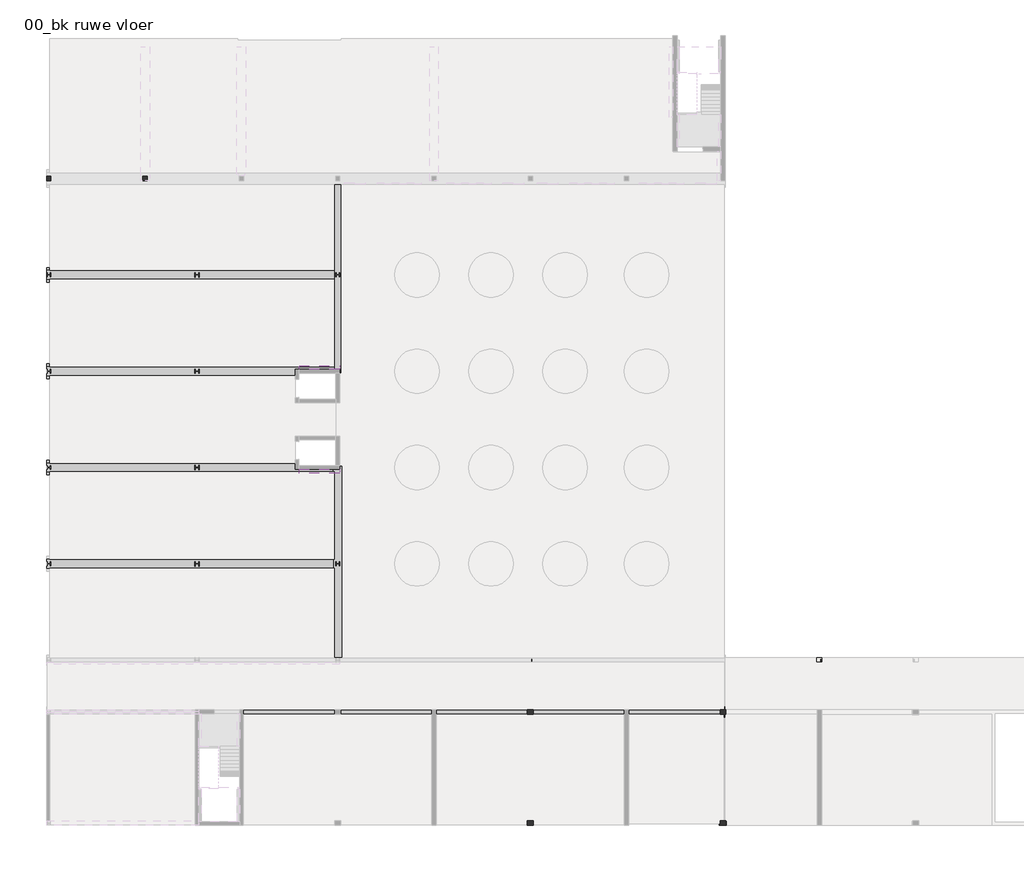
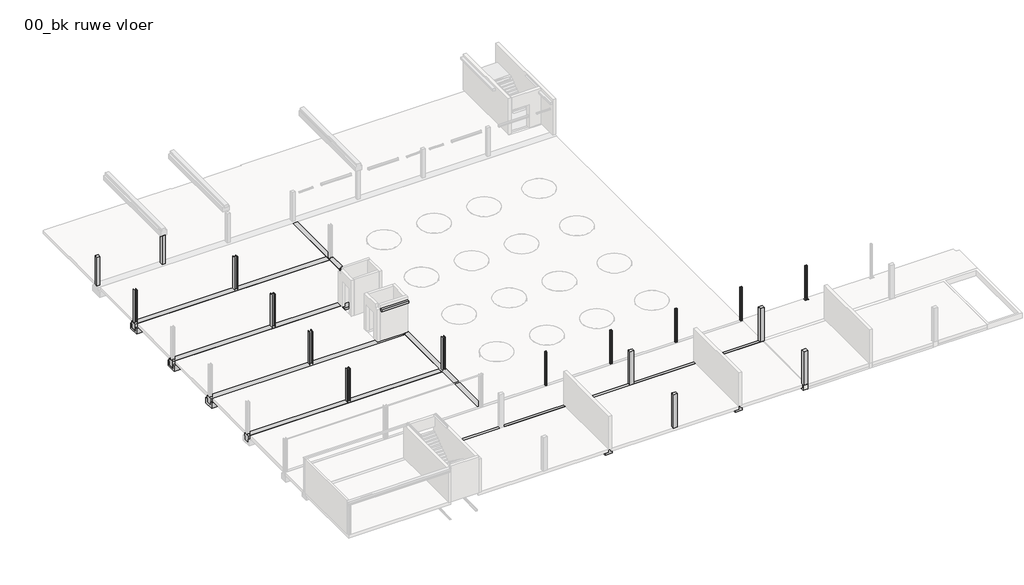
# One storey, part 5 of 6: 17 columns, 14 beams, 2 slabs.
"""IFC4 building model written with IfcOpenShell, lengths in millimetres."""

import ifcopenshell
import ifcopenshell.guid

model = None  # the IFC model being written
_history = None  # IfcOwnerHistory: only IFC2X3 demands one
_inside = {}  # id of a spatial element -> (the spatial element, [elements in it])
_under = {}  # id of a project, library or spatial element -> (it, [spatial elements below it])
_declared = {}  # id of a project -> (the project, [libraries it declares])
_typed = {}  # id of a type object -> (the type object, [elements of that type])
_made_of = {}  # id of a material, layer set ... -> (it, [elements and type objects made of it])


def new_model(schema):
    """Start an empty IFC model of exactly this schema.

    Asked for "IFC4X3", IfcOpenShell would pick the latest addendum, in which some entities
    have other attributes; the version numbers below select the first issue.
    IFC2X3 requires an IfcOwnerHistory on every rooted entity: one is made here for all.
    """
    global model, _history
    if schema == "IFC4X3":
        model = ifcopenshell.file(schema_version=(4, 3, 0, 0))
    else:
        model = ifcopenshell.file(schema=schema)
    _inside.clear()
    _under.clear()
    _declared.clear()
    _typed.clear()
    _made_of.clear()
    _history = None
    if model.schema == "IFC2X3":
        org = make("IfcOrganization", Name="unknown")
        user = make(
            "IfcPersonAndOrganization",
            ThePerson=make("IfcPerson", FamilyName="unknown"),
            TheOrganization=org,
        )
        app = make(
            "IfcApplication",
            ApplicationDeveloper=org,
            Version="unknown",
            ApplicationFullName="unknown",
            ApplicationIdentifier="unknown",
        )
        _history = make(
            "IfcOwnerHistory",
            OwningUser=user,
            OwningApplication=app,
            ChangeAction="ADDED",
            CreationDate=0,
        )
    return model


def make(cls, **values):
    """One entity of the class cls with the attributes given. An attribute that is None is left unset."""
    return model.create_entity(
        cls, **{name: value for name, value in values.items() if value is not None}
    )


def rooted(cls, **values):
    """An entity with a GlobalId (a new one), such as an element, a storey or a relation."""
    return make(cls, GlobalId=ifcopenshell.guid.new(), OwnerHistory=_history, **values)


def si_unit(unit_type, name, prefix=None):
    """IfcSIUnit, for example si_unit("LENGTHUNIT", "METRE", prefix="MILLI")."""
    return make("IfcSIUnit", UnitType=unit_type, Prefix=prefix, Name=name)


def assignment(units):
    """IfcUnitAssignment: the units of a project."""
    return None if units is None else make("IfcUnitAssignment", Units=units)


def point(xyz):
    """IfcCartesianPoint."""
    return None if xyz is None else make("IfcCartesianPoint", Coordinates=xyz)


def direction(xyz):
    """IfcDirection."""
    return None if xyz is None else make("IfcDirection", DirectionRatios=xyz)


def frame(location, z_axis=None, x_axis=None):
    """IfcAxis2Placement3D, a coordinate frame: its origin and axes. An axis left out is left unset."""
    return make(
        "IfcAxis2Placement3D",
        Location=point(location),
        Axis=direction(z_axis),
        RefDirection=direction(x_axis),
    )


def frame_2d(location, x_axis=None):
    """IfcAxis2Placement2D, a coordinate frame in the plane: its origin and x axis."""
    return make(
        "IfcAxis2Placement2D", Location=point(location), RefDirection=direction(x_axis)
    )


def origin():
    """The frame at (0, 0, 0) with its axes left unset."""
    return frame((0.0, 0.0, 0.0))


def place(relative_to, where):
    """IfcLocalPlacement: puts the frame where relative to a parent placement (None: the world)."""
    return make(
        "IfcLocalPlacement", PlacementRelTo=relative_to, RelativePlacement=where
    )


def context(
    kind, dimensions, precision=None, world=None, true_north=None, identifier=None
):
    """IfcGeometricRepresentationContext, for example the 3D "Model" context."""
    return make(
        "IfcGeometricRepresentationContext",
        ContextIdentifier=identifier,
        ContextType=kind,
        CoordinateSpaceDimension=dimensions,
        Precision=precision,
        WorldCoordinateSystem=world,
        TrueNorth=true_north,
    )


def project(units=None, contexts=None):
    """IfcProject with its units and contexts."""
    return rooted(
        "IfcProject",
        Name="project",
        RepresentationContexts=contexts,
        UnitsInContext=assignment(units),
    )


def spatial(cls, under=None, at=None, **own):
    """A site, building, storey or space (cls), placed at a placement, below another one or the project."""
    s = rooted(cls, ObjectPlacement=at, **own)
    if under is not None:
        _under.setdefault(under.id(), (under, []))[1].append(s)
    return s


def polyline(points):
    """IfcPolyline through the points."""
    return make("IfcPolyline", Points=[point(p) for p in points])


def circle_curve(where, radius):
    """IfcCircle in the frame where."""
    return make("IfcCircle", Position=where, Radius=radius)


def trimmed(basis, trim1, trim2, sense, master):
    """IfcTrimmedCurve: the piece of a basis curve between two trims."""
    return make(
        "IfcTrimmedCurve",
        BasisCurve=basis,
        Trim1=trim1,
        Trim2=trim2,
        SenseAgreement=sense,
        MasterRepresentation=master,
    )


def segment(curve, same_sense, transition):
    """IfcCompositeCurveSegment."""
    return make(
        "IfcCompositeCurveSegment",
        Transition=transition,
        SameSense=same_sense,
        ParentCurve=curve,
    )


def composite_curve(segments, self_intersect=None):
    """IfcCompositeCurve: segments joined end to end."""
    return make("IfcCompositeCurve", Segments=segments, SelfIntersect=self_intersect)


def outline(outer, holes=None, kind="AREA"):
    """IfcArbitraryClosedProfileDef: a profile drawn as a closed curve; with holes, ...WithVoids."""
    if holes is None:
        return make("IfcArbitraryClosedProfileDef", ProfileType=kind, OuterCurve=outer)
    return make(
        "IfcArbitraryProfileDefWithVoids",
        ProfileType=kind,
        OuterCurve=outer,
        InnerCurves=holes,
    )


def extrude(swept, where, along, depth):
    """IfcExtrudedAreaSolid: the profile swept, set in the frame where, extruded along a direction by depth."""
    return make(
        "IfcExtrudedAreaSolid",
        SweptArea=swept,
        Position=where,
        ExtrudedDirection=direction(along),
        Depth=depth,
    )


def faces_of(points, faces, orient=None, outer=None):
    """IfcFace entities. A face is a list of loops; a loop is a list of indices into points, from 0.

    orient and outer hold one flag for each loop. By default every Orientation is true, the
    first loop of a face is its IfcFaceOuterBound and the others are IfcFaceBound.
    """
    made = []
    for i, loops in enumerate(faces):
        bounds = []
        for j, loop in enumerate(loops):
            is_outer = j == 0 if outer is None else outer[i][j]
            bounds.append(
                make(
                    "IfcFaceOuterBound" if is_outer else "IfcFaceBound",
                    Bound=make("IfcPolyLoop", Polygon=[points[k] for k in loop]),
                    Orientation=True if orient is None else orient[i][j],
                )
            )
        made.append(make("IfcFace", Bounds=bounds))
    return made


def faceted_brep(points, faces, orient=None, outer=None, voids=None):
    """IfcFacetedBrep: a solid bounded by flat faces; with voids (closed shells), ...WithVoids."""
    shared = [point(p) for p in points]
    hull = make("IfcClosedShell", CfsFaces=faces_of(shared, faces, orient, outer))
    if voids is None:
        return make("IfcFacetedBrep", Outer=hull)
    return make(
        "IfcFacetedBrepWithVoids",
        Outer=hull,
        Voids=[
            make(cls, CfsFaces=faces_of(shared, fs, o, b)) for cls, fs, o, b in voids
        ],
    )


def shape(context_of_items, identifier, shape_type, items):
    """IfcShapeRepresentation: the items that make up one representation, for example the "Body"."""
    return make(
        "IfcShapeRepresentation",
        ContextOfItems=context_of_items,
        RepresentationIdentifier=identifier,
        RepresentationType=shape_type,
        Items=items,
    )


def source(mapping_origin, context_of_items, identifier, shape_type, items):
    """IfcRepresentationMap: a shape defined once, which mapped items show again and again."""
    return make(
        "IfcRepresentationMap",
        MappingOrigin=mapping_origin,
        MappedRepresentation=shape(context_of_items, identifier, shape_type, items),
    )


def transform(
    local_origin,
    x_axis=None,
    y_axis=None,
    z_axis=None,
    scale=None,
    scale2=None,
    scale3=None,
    uniform=True,
):
    """IfcCartesianTransformationOperator3D, or its non-uniform kind. x_axis, y_axis, z_axis: its Axis1, 2, 3."""
    if uniform:
        return make(
            "IfcCartesianTransformationOperator3D",
            Axis1=direction(x_axis),
            Axis2=direction(y_axis),
            LocalOrigin=point(local_origin),
            Scale=scale,
            Axis3=direction(z_axis),
        )
    return make(
        "IfcCartesianTransformationOperator3DnonUniform",
        Axis1=direction(x_axis),
        Axis2=direction(y_axis),
        LocalOrigin=point(local_origin),
        Scale=scale,
        Axis3=direction(z_axis),
        Scale2=scale2,
        Scale3=scale3,
    )


def mapped(mapping_source, mapping_target):
    """IfcMappedItem: shows the shape of a source again, moved by a transform."""
    return make(
        "IfcMappedItem", MappingSource=mapping_source, MappingTarget=mapping_target
    )


def made_of(thing, what):
    """Note that an element or type object is made of a material, layer set ...; save() writes the relation."""
    if what is not None:
        _made_of.setdefault(what.id(), (what, []))[1].append(thing)
    return thing


def element(
    cls,
    number,
    at=None,
    inside=None,
    cuts=None,
    type_object=None,
    material=None,
    context=None,
    identifier="Body",
    shape_type=None,
    held_by="IfcProductDefinitionShape",
    body=None,
    shapes=None,
    **own,
):
    """One element of the class cls, such as IfcWall. Its Tag is "e" and its number.

    at: its placement. inside: the storey or other place that contains it. cuts: it is an
    opening in that element (IfcRelVoidsElement). A single representation is given by context,
    identifier, shape_type and body (its items); several are given by shapes. held_by: the class
    of the entity that holds the representations. save() writes the other relations.
    """
    e = rooted(cls, Tag="e%d" % number, ObjectPlacement=at, **own)
    if body is not None:
        shapes = [shape(context, identifier, shape_type, body)]
    if shapes is not None:
        e.Representation = make(held_by, Representations=shapes)
    if inside is not None:
        _inside.setdefault(inside.id(), (inside, []))[1].append(e)
    if cuts is not None:
        rooted(
            "IfcRelVoidsElement", RelatingBuildingElement=cuts, RelatedOpeningElement=e
        )
    if type_object is not None:
        _typed.setdefault(type_object.id(), (type_object, []))[1].append(e)
    return made_of(e, material)


def aggregate(whole, parts):
    """IfcRelAggregates: a whole, such as a stair, and the parts it consists of."""
    return rooted("IfcRelAggregates", RelatingObject=whole, RelatedObjects=parts)


def save(model, path):
    """Write the relations noted so far, then the file.

    IfcRelAggregates (storeys below a building ...), IfcRelContainedInSpatialStructure (elements
    in a storey), IfcRelDefinesByType, IfcRelAssociatesMaterial and IfcRelDeclares: one each for
    every whole, place, type object, material and project.
    """
    for whole, parts in _under.values():
        aggregate(whole, parts)
    for where, things in _inside.values():
        rooted(
            "IfcRelContainedInSpatialStructure",
            RelatedElements=things,
            RelatingStructure=where,
        )
    for kind, things in _typed.values():
        rooted("IfcRelDefinesByType", RelatedObjects=things, RelatingType=kind)
    for what, things in _made_of.values():
        rooted("IfcRelAssociatesMaterial", RelatedObjects=things, RelatingMaterial=what)
    for by, libraries in _declared.values():
        rooted("IfcRelDeclares", RelatingContext=by, RelatedDefinitions=libraries)
    model.write(path)


def column_d8346d76(model_context):
    return source(origin(), model_context, "Body", "SweptSolid", [
        extrude(outline(composite_curve([segment(trimmed(circle_curve(frame_2d((60.0, 60.0)), 20.0), [point((60.0, 80.0))], [point((80.0, 60.0))], False, "CARTESIAN"), True, "CONTINUOUS"), segment(polyline([(80.0, 60.0), (80.0, -60.0)]), True, "CONTINUOUS"), segment(trimmed(circle_curve(frame_2d((60.0, -60.0)), 20.0), [point((80.0, -60.0))], [point((60.0, -80.0))], False, "CARTESIAN"), True, "CONTINUOUS"), segment(polyline([(60.0, -80.0), (-60.0, -80.0)]), True, "CONTINUOUS"), segment(trimmed(circle_curve(frame_2d((-60.0, -60.0)), 20.0), [point((-60.0, -80.0))], [point((-80.0, -60.0))], False, "CARTESIAN"), True, "CONTINUOUS"), segment(polyline([(-80.0, -60.0), (-80.0, 60.0)]), True, "CONTINUOUS"), segment(trimmed(circle_curve(frame_2d((-60.0, 60.0)), 20.0), [point((-80.0, 60.0))], [point((-60.0, 80.0))], False, "CARTESIAN"), True, "CONTINUOUS"), segment(polyline([(-60.0, 80.0), (60.0, 80.0)]), True, "CONTINUOUS")], self_intersect=False), holes=[composite_curve([segment(polyline([(60.0, 72.0), (-60.0, 72.0)]), True, "CONTINUOUS"), segment(trimmed(circle_curve(frame_2d((-60.0, 60.0)), 12.0), [point((-60.0, 72.0))], [point((-72.0, 60.0))], True, "CARTESIAN"), True, "CONTINUOUS"), segment(polyline([(-72.0, 60.0), (-72.0, -60.0)]), True, "CONTINUOUS"), segment(trimmed(circle_curve(frame_2d((-60.0, -60.0)), 12.0), [point((-72.0, -60.0))], [point((-60.0, -72.0))], True, "CARTESIAN"), True, "CONTINUOUS"), segment(polyline([(-60.0, -72.0), (60.0, -72.0)]), True, "CONTINUOUS"), segment(trimmed(circle_curve(frame_2d((60.0, -60.0)), 12.0), [point((60.0, -72.0))], [point((72.0, -60.0))], True, "CARTESIAN"), True, "CONTINUOUS"), segment(polyline([(72.0, -60.0), (72.0, 60.0)]), True, "CONTINUOUS"), segment(trimmed(circle_curve(frame_2d((60.0, 60.0)), 12.0), [point((72.0, 60.0))], [point((60.0, 72.0))], True, "CARTESIAN"), True, "CONTINUOUS")], self_intersect=False)]), frame((0.0, 0.0, -40.0), z_axis=(0.0, 0.0, 1.0), x_axis=(1.0, 0.0, 0.0)), (0.0, 0.0, 1.0), 3510.0),
    ])


model = new_model("IFC4")

# Units and contexts
model_context = context("Model", 3, world=origin())
ifc_project = project(units=[si_unit("LENGTHUNIT", "METRE", prefix="MILLI")], contexts=[model_context])

# Site, building, storey
site = spatial("IfcSite", under=ifc_project)
building = spatial("IfcBuilding", under=site)
storey = spatial("IfcBuildingStorey", under=building, Name="00_bk ruwe vloer", Elevation=-70.0)

# Beams
placement = place(None, origin())
element("IfcBeam", 1, ObjectType="NLRS_28_SF_LIB_balk dubbele sponning beton prefab-CWV-MMBC-SRP_gen_rsf : balk beton prefab_gen__bxh 700x700 met inkassing bxh 200x320", at=placement, inside=storey, context=model_context, shape_type="Brep", body=[
    faceted_brep([(52150.0, 7650.0, -70.0), (52150.0, 7350.0, -70.0), (52150.0, 7350.0, -390.0), (52150.0, 7150.0, -390.0), (52150.0, 7150.0, -770.0), (52150.0, 7850.0, -770.0), (52150.0, 7850.0, -390.0), (52150.0, 7650.0, -390.0), (52090.0, 7650.0, -70.0), (51800.0, 7650.0, -70.0), (39200.0, 7650.0, -70.0), (38800.0, 7650.0, -70.0), (26200.0, 7650.0, -70.0), (25800.0, 7650.0, -70.0), (19625.0, 7650.0, -70.0), (19375.0, 7650.0, -70.0), (19375.0, 7400.0, -70.0), (19375.0, 7350.0, -70.0), (25800.0, 7350.0, -70.0), (26200.0, 7350.0, -70.0), (32350.0, 7350.0, -70.0), (32650.0, 7350.0, -70.0), (38800.0, 7350.0, -70.0), (39200.0, 7350.0, -70.0), (45350.0, 7350.0, -70.0), (45650.0, 7350.0, -70.0), (51800.0, 7350.0, -70.0), (52050.0, 7350.0, -70.0), (19375.0, 7350.0, -390.0), (19625.0, 7350.0, -390.0), (32350.0, 7350.0, -390.0), (32650.0, 7350.0, -390.0), (45350.0, 7350.0, -390.0), (45650.0, 7350.0, -390.0), (52050.0, 7350.0, -390.0), (19625.0, 7175.0, -390.0), (19625.0, 7150.0, -390.0), (32150.0, 7150.0, -390.0), (32175.0, 7150.0, -390.0), (32350.0, 7150.0, -390.0), (32650.0, 7150.0, -390.0), (32825.0, 7150.0, -390.0), (32850.0, 7150.0, -390.0), (45150.0, 7150.0, -390.0), (45175.0, 7150.0, -390.0), (45350.0, 7150.0, -390.0), (45650.0, 7150.0, -390.0), (45825.0, 7150.0, -390.0), (45850.0, 7150.0, -390.0), (51850.0, 7150.0, -390.0), (51875.0, 7150.0, -390.0), (52050.0, 7150.0, -390.0), (19625.0, 7150.0, -770.0), (32150.0, 7150.0, -770.0), (32850.0, 7150.0, -770.0), (45150.0, 7150.0, -770.0), (45850.0, 7150.0, -770.0), (51850.0, 7150.0, -770.0), (19625.0, 7650.0, -770.0), (19375.0, 7650.0, -770.0), (19375.0, 7850.0, -770.0), (51850.0, 7850.0, -770.0), (19375.0, 7850.0, -390.0), (51850.0, 7850.0, -390.0), (51875.0, 7850.0, -390.0), (52090.0, 7850.0, -390.0), (19375.0, 7825.0, -390.0), (19375.0, 7650.0, -390.0), (19625.0, 7650.0, -390.0), (52090.0, 7650.0, -390.0), (19625.0, 7650.0, -390.0)], [[[0, 1, 2, 3, 4, 5, 6, 7]], [[1, 0, 8, 9, 10, 11, 12, 13, 14, 15, 16, 17, 18, 19, 20, 21, 22, 23, 24, 25, 26, 27]], [[2, 1, 27, 26, 25, 24, 23, 22, 21, 20, 19, 18, 17, 28, 29, 30, 31, 32, 33, 34]], [[3, 2, 34, 33, 32, 31, 30, 29, 35, 36, 37, 38, 39, 40, 41, 42, 43, 44, 45, 46, 47, 48, 49, 50, 51]], [[4, 3, 51, 50, 49, 48, 47, 46, 45, 44, 43, 42, 41, 40, 39, 38, 37, 36, 52, 53, 54, 55, 56, 57]], [[5, 4, 57, 56, 55, 54, 53, 52, 58, 59, 60, 61]], [[6, 5, 61, 60, 62, 63, 64, 65]], [[7, 6, 65, 64, 63, 62, 66, 67, 68, 69]], [[0, 7, 69, 68, 67, 15, 14, 13, 12, 11, 10, 9, 8]], [[17, 16, 15, 67, 28]], [[29, 70, 58, 52, 36, 35]], [[67, 70, 29, 28]], [[70, 67, 59, 58]], [[62, 60, 59, 67, 66]]]),
])
element("IfcBeam", 2, ObjectType="NLRS_28_SF_LIB_balk dubbele sponning beton ihwg-CWV-MMBC-SRP_gen_rsf : balk beton ihwg_gen__bxh 1000x900 met inkassing bxh 200x320", at=placement, inside=storey, context=model_context, shape_type="Brep", body=[
    faceted_brep([(6350.0, 17200.0, -70.0), (6350.0, 17800.0, -70.0), (6350.0, 17800.0, -390.0), (6350.0, 17800.0, -770.0), (6350.0, 17200.0, -770.0), (6350.0, 17200.0, -390.0), (6550.0, 17200.0, -70.0), (25700.0, 17200.0, -70.0), (25700.0, 17800.0, -70.0), (6550.0, 17800.0, -70.0), (25500.0, 17200.0, -770.0), (25500.0, 17200.0, -390.0), (25550.0, 17200.0, -390.0), (25700.0, 17200.0, -390.0), (25700.0, 17800.0, -390.0), (25550.0, 17800.0, -390.0), (25500.0, 17800.0, -390.0), (25500.0, 17800.0, -770.0)], [[[0, 1, 2, 3, 4, 5]], [[1, 0, 6, 7, 8, 9]], [[0, 5, 4, 10, 11, 12, 13, 7, 6]], [[3, 2, 1, 9, 8, 14, 15, 16, 17]], [[4, 3, 17, 10]], [[16, 11, 10, 17]], [[14, 13, 12, 11, 16, 15]], [[13, 14, 8, 7]]]),
])
element("IfcBeam", 3, ObjectType="NLRS_28_SF_LIB_balk dubbele sponning beton ihwg-CWV-MMBC-SRP_gen_rsf : balk beton ihwg_gen__bxh 1000x900 met inkassing bxh 200x320", at=placement, inside=storey, context=model_context, shape_type="Brep", body=[
    faceted_brep([(6350.0, 23700.0, -70.0), (6350.0, 24300.0, -70.0), (6350.0, 24300.0, -390.0), (6350.0, 24300.0, -770.0), (6350.0, 23700.0, -770.0), (6350.0, 23700.0, -390.0), (6550.0, 23700.0, -70.0), (25700.0, 23700.0, -70.0), (25700.0, 23875.0, -70.0), (23375.0, 23875.0, -70.0), (23125.0, 23875.0, -70.0), (23125.0, 24300.0, -70.0), (6550.0, 24300.0, -70.0), (25500.0, 23700.0, -770.0), (25500.0, 23700.0, -390.0), (25550.0, 23700.0, -390.0), (25700.0, 23700.0, -390.0), (23125.0, 24300.0, -390.0), (23125.0, 24300.0, -770.0), (23125.0, 23875.0, -770.0), (23375.0, 23875.0, -770.0), (25500.0, 23875.0, -770.0), (25500.0, 23875.0, -390.0), (25700.0, 23875.0, -390.0)], [[[0, 1, 2, 3, 4, 5]], [[1, 0, 6, 7, 8, 9, 10, 11, 12]], [[0, 5, 4, 13, 14, 15, 16, 7, 6]], [[3, 2, 1, 12, 11, 17, 18]], [[4, 3, 18, 19, 20, 21, 13]], [[17, 11, 10, 19, 18]], [[22, 14, 13, 21]], [[14, 22, 23, 16, 15]], [[16, 23, 8, 7]], [[19, 10, 9, 8, 23, 22, 21, 20]]]),
])
element("IfcBeam", 4, ObjectType="NLRS_28_SF_LIB_balk dubbele sponning beton ihwg-CWV-MMBC-SRP_gen_rsf : balk beton ihwg_gen__bxh 1000x900 met inkassing bxh 200x320", at=placement, inside=storey, context=model_context, shape_type="Brep", body=[
    faceted_brep([(25750.0, 30800.0, -390.0), (25750.0, 30800.0, -70.0), (25750.0, 30625.0, -70.0), (25750.0, 30625.0, -390.0), (6350.0, 30200.0, -70.0), (6350.0, 30800.0, -70.0), (6350.0, 30800.0, -390.0), (6350.0, 30800.0, -770.0), (6350.0, 30200.0, -770.0), (6350.0, 30200.0, -390.0), (6550.0, 30200.0, -70.0), (23125.0, 30200.0, -70.0), (23375.0, 30200.0, -70.0), (23375.0, 30375.0, -70.0), (23375.0, 30625.0, -70.0), (6550.0, 30800.0, -70.0), (23375.0, 30200.0, -770.0), (23375.0, 30200.0, -390.0), (25550.0, 30800.0, -390.0), (25550.0, 30800.0, -770.0), (25550.0, 30625.0, -770.0), (23375.0, 30625.0, -770.0), (25550.0, 30625.0, -390.0)], [[[0, 1, 2, 3]], [[4, 5, 6, 7, 8, 9]], [[5, 4, 10, 11, 12, 13, 14, 2, 1, 15]], [[4, 9, 8, 16, 17, 12, 11, 10]], [[1, 0, 18, 19, 7, 6, 5, 15]], [[7, 19, 20, 21, 16, 8]], [[14, 21, 20, 22, 3, 2]], [[21, 14, 13, 12, 17, 16]], [[18, 22, 20, 19]], [[22, 18, 0, 3]]]),
])
element("IfcBeam", 5, ObjectType="NLRS_28_SF_LIB_balk dubbele sponning beton ihwg-CWV-MMBC-SRP_gen_rsf : balk beton ihwg_gen__bxh 1000x900 met inkassing bxh 200x320", at=placement, inside=storey, context=model_context, shape_type="Brep", body=[
    faceted_brep([(6350.0, 36700.0, -70.0), (6350.0, 37300.0, -70.0), (6350.0, 37300.0, -390.0), (6350.0, 37300.0, -770.0), (6350.0, 36700.0, -770.0), (6350.0, 36700.0, -390.0), (6550.0, 36700.0, -70.0), (25750.0, 36700.0, -70.0), (25750.0, 37300.0, -70.0), (6550.0, 37300.0, -70.0), (25550.0, 36700.0, -770.0), (25550.0, 36700.0, -390.0), (25750.0, 36700.0, -390.0), (25550.0, 37300.0, -770.0), (25750.0, 37300.0, -390.0), (25550.0, 37300.0, -390.0)], [[[0, 1, 2, 3, 4, 5]], [[1, 0, 6, 7, 8, 9]], [[4, 10, 11, 12, 7, 6, 0, 5]], [[13, 3, 2, 1, 9, 8, 14, 15]], [[3, 13, 10, 4]], [[15, 11, 10, 13]], [[11, 15, 14, 12]], [[12, 14, 8, 7]]]),
])
element("IfcBeam", 6, ObjectType="NLRS_28_SF_LIB_balkbodem beton prefab-CWV-MMBC-SRP_gen_rsf : balkbodem beton prefab_gen__bxhxdk 1000x580x200", at=placement, inside=storey, context=model_context, shape_type="Brep", body=[
    faceted_brep([(25550.0, 36500.0, -390.0), (25550.0, 36500.0, -970.0), (25550.0, 37500.0, -970.0), (25550.0, 37500.0, -390.0), (25550.0, 37300.0, -390.0), (25550.0, 37300.0, -770.0), (25550.0, 36700.0, -770.0), (25550.0, 36700.0, -390.0), (6350.0, 36500.0, -390.0), (6350.0, 36700.0, -390.0), (6350.0, 36700.0, -770.0), (6350.0, 37300.0, -770.0), (6350.0, 37300.0, -390.0), (6350.0, 37500.0, -390.0), (6350.0, 37500.0, -970.0), (6350.0, 36500.0, -970.0), (6650.0, 36500.0, -390.0), (6550.0, 36500.0, -390.0), (6650.0, 36500.0, -970.0), (6650.0, 37500.0, -970.0), (6550.0, 37500.0, -390.0), (6650.0, 37500.0, -390.0), (6550.0, 37300.0, -390.0), (6550.0, 36700.0, -390.0)], [[[0, 1, 2, 3, 4, 5, 6, 7]], [[8, 9, 10, 11, 12, 13, 14, 15]], [[1, 0, 16, 17, 8, 15, 18]], [[2, 1, 18, 15, 14, 19]], [[3, 2, 19, 14, 13, 20, 21]], [[4, 3, 21, 20, 13, 12, 22]], [[5, 4, 22, 12, 11]], [[6, 5, 11, 10]], [[7, 6, 10, 9, 23]], [[0, 7, 23, 9, 8, 17, 16]]]),
])
element("IfcBeam", 7, ObjectType="NLRS_28_SF_LIB_balkbodem beton prefab-CWV-MMBC-SRP_gen_rsf : balkbodem beton prefab_gen__bxhxdk 1000x580x200", at=placement, inside=storey, context=model_context, shape_type="Brep", body=[
    faceted_brep([(25550.0, 31000.0, -970.0), (25550.0, 31000.0, -390.0), (25550.0, 30800.0, -390.0), (25550.0, 30800.0, -770.0), (25550.0, 30625.0, -770.0), (25550.0, 30625.0, -970.0), (6350.0, 30000.0, -390.0), (6350.0, 30200.0, -390.0), (6350.0, 30200.0, -770.0), (6350.0, 30800.0, -770.0), (6350.0, 30800.0, -390.0), (6350.0, 31000.0, -390.0), (6350.0, 31000.0, -970.0), (6350.0, 30000.0, -970.0), (6650.0, 30000.0, -970.0), (23125.0, 30000.0, -970.0), (23375.0, 30000.0, -970.0), (23375.0, 30000.0, -390.0), (23125.0, 30000.0, -390.0), (6650.0, 30000.0, -390.0), (6550.0, 30000.0, -390.0), (6650.0, 31000.0, -970.0), (23375.0, 30625.0, -970.0), (6550.0, 31000.0, -390.0), (6650.0, 31000.0, -390.0), (6550.0, 30800.0, -390.0), (23375.0, 30200.0, -770.0), (23375.0, 30625.0, -770.0), (6550.0, 30200.0, -390.0), (23125.0, 30200.0, -390.0), (23375.0, 30200.0, -390.0)], [[[0, 1, 2, 3, 4, 5]], [[6, 7, 8, 9, 10, 11, 12, 13]], [[6, 13, 14, 15, 16, 17, 18, 19, 20]], [[13, 12, 21, 0, 5, 22, 16, 15, 14]], [[1, 0, 21, 12, 11, 23, 24]], [[2, 1, 24, 23, 11, 10, 25]], [[3, 2, 25, 10, 9]], [[9, 8, 26, 27, 4, 3]], [[8, 7, 28, 29, 30, 26]], [[7, 6, 20, 19, 18, 17, 30, 29, 28]], [[27, 22, 5, 4]], [[17, 16, 22, 27, 26, 30]]]),
])
element("IfcBeam", 8, ObjectType="NLRS_28_SF_LIB_balkbodem beton prefab-CWV-MMBC-SRP_gen_rsf : balkbodem beton prefab_gen__bxhxdk 1000x580x200", at=placement, inside=storey, context=model_context, shape_type="Brep", body=[
    faceted_brep([(25550.0, 23500.0, -390.0), (25550.0, 23500.0, -970.0), (25550.0, 23875.0, -970.0), (25550.0, 23875.0, -770.0), (25550.0, 23700.0, -770.0), (25550.0, 23700.0, -390.0), (6350.0, 23500.0, -390.0), (6350.0, 23700.0, -390.0), (6350.0, 23700.0, -770.0), (6350.0, 24300.0, -770.0), (6350.0, 24300.0, -390.0), (6350.0, 24500.0, -390.0), (6350.0, 24500.0, -970.0), (6350.0, 23500.0, -970.0), (25500.0, 23500.0, -390.0), (6650.0, 23500.0, -390.0), (6550.0, 23500.0, -390.0), (6650.0, 23500.0, -970.0), (25500.0, 23500.0, -970.0), (6650.0, 24500.0, -970.0), (23125.0, 24500.0, -970.0), (23375.0, 24500.0, -970.0), (23375.0, 23875.0, -970.0), (6550.0, 24500.0, -390.0), (6650.0, 24500.0, -390.0), (23125.0, 24500.0, -390.0), (23375.0, 24500.0, -390.0), (6550.0, 24300.0, -390.0), (23125.0, 24300.0, -390.0), (23375.0, 24300.0, -390.0), (23125.0, 24300.0, -770.0), (23375.0, 24300.0, -770.0), (25500.0, 23700.0, -770.0), (25500.0, 23875.0, -770.0), (23375.0, 23875.0, -770.0), (6550.0, 23700.0, -390.0), (25500.0, 23700.0, -390.0)], [[[0, 1, 2, 3, 4, 5]], [[6, 7, 8, 9, 10, 11, 12, 13]], [[1, 0, 14, 15, 16, 6, 13, 17, 18]], [[13, 12, 19, 20, 21, 22, 2, 1, 18, 17]], [[12, 11, 23, 24, 25, 26, 21, 20, 19]], [[11, 10, 27, 28, 29, 26, 25, 24, 23]], [[10, 9, 30, 31, 29, 28, 27]], [[9, 8, 32, 4, 3, 33, 34, 31, 30]], [[5, 4, 32, 8, 7, 35, 36]], [[0, 5, 36, 35, 7, 6, 16, 15, 14]], [[22, 34, 33, 3, 2]], [[21, 26, 29, 31, 34, 22]]]),
])
element("IfcBeam", 9, ObjectType="NLRS_28_SF_LIB_balk dubbele sponning beton ihwg-CWV-MMBC-SRP_gen_rsf : balk beton ihwg_gen__bxh 900x900 met inkassing bxh 200x320", at=placement, inside=storey, context=model_context, shape_type="Brep", body=[
    faceted_brep([(25750.0, 43100.0, -70.0), (26250.0, 43100.0, -70.0), (26250.0, 43100.0, -390.0), (25750.0, 43100.0, -390.0), (25750.0, 30375.0, -70.0), (25750.0, 30375.0, -390.0), (25550.0, 30375.0, -390.0), (25550.0, 30375.0, -970.0), (25875.0, 30375.0, -970.0), (25875.0, 30375.0, -390.0), (26125.0, 30375.0, -390.0), (26125.0, 30375.0, -970.0), (26450.0, 30375.0, -970.0), (26450.0, 30375.0, -390.0), (26425.0, 30375.0, -390.0), (26250.0, 30375.0, -390.0), (26250.0, 30375.0, -70.0), (25750.0, 37300.0, -70.0), (25750.0, 36700.0, -70.0), (25750.0, 30800.0, -70.0), (25750.0, 30625.0, -70.0), (26250.0, 42900.0, -390.0), (26450.0, 42900.0, -390.0), (26425.0, 42900.0, -390.0), (26450.0, 42900.0, -970.0), (26125.0, 30625.0, -970.0), (25875.0, 30625.0, -970.0), (25550.0, 30625.0, -970.0), (25550.0, 36500.0, -970.0), (25550.0, 37500.0, -970.0), (25550.0, 42900.0, -970.0), (25550.0, 30625.0, -390.0), (25550.0, 30800.0, -390.0), (25550.0, 36500.0, -390.0), (25550.0, 36700.0, -390.0), (25550.0, 37300.0, -390.0), (25550.0, 37500.0, -390.0), (25550.0, 42900.0, -390.0), (25750.0, 30625.0, -390.0), (25750.0, 30800.0, -390.0), (25750.0, 36700.0, -390.0), (25750.0, 37300.0, -390.0), (25750.0, 42900.0, -390.0), (26125.0, 30625.0, -390.0), (25875.0, 30625.0, -390.0)], [[[0, 1, 2, 3]], [[4, 5, 6, 7, 8, 9, 10, 11, 12, 13, 14, 15, 16]], [[1, 0, 17, 18, 19, 20, 4, 16]], [[2, 1, 16, 15, 21]], [[21, 15, 14, 13, 22, 23]], [[13, 12, 24, 22]], [[12, 11, 25, 26, 8, 7, 27, 28, 29, 30, 24]], [[7, 6, 31, 32, 33, 34, 35, 36, 37, 30, 29, 28, 27]], [[6, 5, 38, 39, 40, 41, 42, 37, 36, 35, 34, 33, 32, 31]], [[0, 3, 42, 41, 40, 39, 38, 5, 4, 20, 19, 18, 17]], [[3, 2, 21, 42]], [[22, 24, 30, 37, 42, 21, 23]], [[10, 43, 25, 11]], [[26, 44, 9, 8]], [[43, 44, 26, 25]], [[44, 43, 10, 9]]]),
])
element("IfcBeam", 10, ObjectType="NLRS_28_SF_LIB_balk dubbele sponning beton ihwg-CWV-MMBC-SRP_gen_rsf : balk beton ihwg_gen__bxh 1000x900 met inkassing bxh 200x320", at=placement, inside=storey, context=model_context, shape_type="Brep", body=[
    faceted_brep([(26300.0, 24125.0, -70.0), (26300.0, 24125.0, -390.0), (26425.0, 24125.0, -390.0), (26500.0, 24125.0, -390.0), (26500.0, 24125.0, -970.0), (26125.0, 24125.0, -970.0), (26125.0, 24125.0, -390.0), (25875.0, 24125.0, -390.0), (25875.0, 24125.0, -70.0), (26300.0, 11150.0, -390.0), (26300.0, 11150.0, -70.0), (25750.0, 11150.0, -70.0), (25750.0, 11150.0, -390.0), (25875.0, 23875.0, -70.0), (25700.0, 23875.0, -70.0), (25700.0, 23700.0, -70.0), (25750.0, 23700.0, -70.0), (25750.0, 17800.0, -70.0), (25700.0, 17800.0, -70.0), (25700.0, 17200.0, -70.0), (25750.0, 17200.0, -70.0), (26300.0, 11350.0, -390.0), (26425.0, 11350.0, -390.0), (26500.0, 11350.0, -390.0), (26500.0, 11350.0, -970.0), (26125.0, 23875.0, -970.0), (25500.0, 11350.0, -970.0), (25500.0, 17000.0, -970.0), (25550.0, 17000.0, -970.0), (25550.0, 18000.0, -970.0), (25500.0, 18000.0, -970.0), (25500.0, 23500.0, -970.0), (25550.0, 23500.0, -970.0), (25550.0, 23875.0, -970.0), (25500.0, 23875.0, -390.0), (25500.0, 23875.0, -770.0), (25500.0, 23700.0, -770.0), (25500.0, 23700.0, -390.0), (25750.0, 11350.0, -390.0), (25750.0, 17200.0, -390.0), (25700.0, 17200.0, -390.0), (25700.0, 17800.0, -390.0), (25750.0, 17800.0, -390.0), (25750.0, 23700.0, -390.0), (25700.0, 23700.0, -390.0), (25700.0, 23875.0, -390.0), (25550.0, 23700.0, -390.0), (25550.0, 23500.0, -390.0), (25500.0, 23500.0, -390.0), (25500.0, 18000.0, -390.0), (25550.0, 18000.0, -390.0), (25550.0, 17800.0, -390.0), (25500.0, 17800.0, -390.0), (25500.0, 17200.0, -390.0), (25550.0, 17200.0, -390.0), (25550.0, 17000.0, -390.0), (25500.0, 17000.0, -390.0), (25500.0, 11350.0, -390.0), (25550.0, 23700.0, -770.0), (25550.0, 23875.0, -770.0), (25550.0, 17200.0, -770.0), (25550.0, 17800.0, -770.0), (25500.0, 17800.0, -770.0), (25500.0, 17200.0, -770.0), (25875.0, 23875.0, -390.0), (26125.0, 23875.0, -390.0)], [[[0, 1, 2, 3, 4, 5, 6, 7, 8]], [[9, 10, 11, 12]], [[10, 0, 8, 13, 14, 15, 16, 17, 18, 19, 20, 11]], [[1, 0, 10, 9, 21]], [[1, 21, 22, 23, 3, 2]], [[4, 3, 23, 24]], [[25, 5, 4, 24, 26, 27, 28, 29, 30, 31, 32, 33]], [[34, 35, 36, 37]], [[38, 39, 40, 41, 42, 43, 44, 45, 34, 37, 46, 47, 48, 49, 50, 51, 52, 53, 54, 55, 56, 57]], [[44, 15, 14, 45]], [[24, 23, 22, 21, 38, 57, 26]], [[12, 38, 21, 9]], [[32, 47, 46, 58, 59, 33]], [[47, 32, 31, 48]], [[58, 46, 37, 36]], [[28, 55, 54, 60, 61, 51, 50, 29]], [[55, 28, 27, 56]], [[29, 50, 49, 30]], [[51, 61, 62, 52]], [[60, 54, 53, 63]], [[20, 39, 38, 12, 11]], [[39, 20, 19, 40]], [[43, 42, 17, 16]], [[17, 42, 41, 18]], [[43, 16, 15, 44]], [[45, 14, 13, 64, 65, 25, 33, 59, 35, 34]], [[25, 65, 6, 5]], [[65, 64, 7, 6]], [[58, 36, 35, 59]], [[61, 60, 63, 62]], [[48, 31, 30, 49]], [[53, 52, 62, 63]], [[26, 57, 56, 27]], [[40, 19, 18, 41]], [[13, 8, 7, 64]]]),
])
element("IfcBeam", 11, ObjectType="NLRS_28_SF_LIB_balk dubbele sponning beton prefab-CWV-MMBC-SRP_gen_rsf : balk beton prefab_gen__bxh 700x700 met inkassing bxh 200x320", at=placement, inside=storey, context=model_context, shape_type="Brep", body=[
    faceted_brep([(32650.0, 7350.0, -70.0), (32350.0, 7350.0, -70.0), (32350.0, 150.0, -70.0), (32650.0, 150.0, -70.0), (32350.0, 7350.0, -390.0), (32350.0, 7150.0, -390.0), (32350.0, 150.0, -390.0), (32850.0, 7150.0, -390.0), (32825.0, 7150.0, -390.0), (32650.0, 7150.0, -390.0), (32650.0, 150.0, -390.0), (32850.0, 150.0, -390.0), (32150.0, 7150.0, -390.0), (32150.0, 7150.0, -770.0), (32150.0, 150.0, -770.0), (32150.0, 150.0, -390.0), (32850.0, 7150.0, -770.0), (32850.0, 150.0, -770.0), (32650.0, 7350.0, -390.0), (32175.0, 7150.0, -390.0)], [[[0, 1, 2, 3]], [[1, 4, 5, 6, 2]], [[7, 8, 9, 10, 11]], [[12, 13, 14, 15]], [[13, 16, 17, 14]], [[16, 7, 11, 17]], [[18, 0, 3, 10, 9]], [[1, 0, 18, 4]], [[5, 4, 18, 9]], [[13, 12, 19, 5, 9, 8, 7, 16]], [[19, 12, 15, 6, 5]], [[3, 2, 6, 15, 14, 17, 11, 10]]]),
])
element("IfcBeam", 12, ObjectType="NLRS_28_SF_LIB_balk dubbele sponning beton prefab-CWV-MMBC-SRP_gen_rsf : balk beton prefab_gen__bxh 700x700 met inkassing bxh 200x320", at=placement, inside=storey, context=model_context, shape_type="Brep", body=[
    faceted_brep([(45650.0, 7350.0, -70.0), (45350.0, 7350.0, -70.0), (45350.0, 150.0, -70.0), (45650.0, 150.0, -70.0), (45350.0, 7350.0, -390.0), (45350.0, 7150.0, -390.0), (45350.0, 150.0, -390.0), (45850.0, 7150.0, -390.0), (45825.0, 7150.0, -390.0), (45650.0, 7150.0, -390.0), (45650.0, 150.0, -390.0), (45850.0, 150.0, -390.0), (45150.0, 7150.0, -390.0), (45150.0, 7150.0, -770.0), (45150.0, 150.0, -770.0), (45150.0, 150.0, -390.0), (45850.0, 7150.0, -770.0), (45850.0, 150.0, -770.0), (45650.0, 7350.0, -390.0), (45175.0, 7150.0, -390.0)], [[[0, 1, 2, 3]], [[1, 4, 5, 6, 2]], [[7, 8, 9, 10, 11]], [[12, 13, 14, 15]], [[13, 16, 17, 14]], [[16, 7, 11, 17]], [[18, 0, 3, 10, 9]], [[1, 0, 18, 4]], [[5, 4, 18, 9]], [[13, 12, 19, 5, 9, 8, 7, 16]], [[19, 12, 15, 6, 5]], [[3, 2, 6, 15, 14, 17, 11, 10]]]),
])
element("IfcBeam", 13, ObjectType="NLRS_22_SF_LIB_oplegnok beton prefab framing-CWV-MMBPC-SRP_gen_rsf : oplegnok beton prefab_gen__bxh 250x250/220", at=placement, inside=storey, context=model_context, shape_type="Brep", body=[
    faceted_brep([(23395.0, 23625.0, 3400.0), (23395.0, 23795.0, 3400.0), (23395.0, 23825.0, 3400.0), (23395.0, 23875.0, 3400.0), (23395.0, 23875.0, 3150.0), (23395.0, 23625.0, 3180.0), (26125.0, 23625.0, 3400.0), (26125.0, 23625.0, 3180.0), (26125.0, 23875.0, 3150.0), (26125.0, 23875.0, 3400.0), (26125.0, 23795.0, 3400.0)], [[[0, 1, 2, 3, 4, 5]], [[6, 7, 8, 9, 10]], [[3, 2, 1, 0, 6, 10, 9]], [[4, 3, 9, 8]], [[0, 5, 7, 6]], [[5, 4, 8, 7]]]),
])
element("IfcBeam", 14, ObjectType="NLRS_22_SF_LIB_oplegnok beton prefab framing-CWV-MMBPC-SRP_gen_rsf : oplegnok beton prefab_gen__bxh 250x250/220", at=placement, inside=storey, context=model_context, shape_type="Brep", body=[
    faceted_brep([(23395.0, 30875.0, 3400.0), (23395.0, 30875.0, 3180.0), (23395.0, 30625.0, 3150.0), (23395.0, 30625.0, 3400.0), (23395.0, 30652.0, 3400.0), (23395.0, 30705.0, 3400.0), (26125.0, 30875.0, 3400.0), (26125.0, 30705.0, 3400.0), (26125.0, 30625.0, 3400.0), (26125.0, 30625.0, 3150.0), (26125.0, 30875.0, 3180.0)], [[[0, 1, 2, 3, 4, 5]], [[6, 7, 8, 9, 10]], [[3, 8, 7, 6, 0, 5, 4]], [[2, 9, 8, 3]], [[0, 6, 10, 1]], [[1, 10, 9, 2]]]),
])

# Columns
element("IfcColumn", 15, ObjectType="NLRS_28_SCO_TLB_stalen kolom HEA-BCPG-MMBS-SRP_gen_rsf : stalen kolom_gen__HEA 260", at=placement, inside=storey, context=model_context, shape_type="SweptSolid", body=[
    extrude(outline(composite_curve([segment(polyline([(6375.0, 37130.0), (6387.5, 37130.0), (6387.5, 37027.75)]), True, "CONTINUOUS"), segment(trimmed(circle_curve(frame_2d((6411.5, 37027.75)), 24.0), [point((6387.5, 37027.75))], [point((6411.5, 37003.75))], True, "CARTESIAN"), True, "CONTINUOUS"), segment(polyline([(6411.5, 37003.75), (6588.5, 37003.75)]), True, "CONTINUOUS"), segment(trimmed(circle_curve(frame_2d((6588.5, 37027.75)), 24.0), [point((6588.5, 37003.75))], [point((6612.5, 37027.75))], True, "CARTESIAN"), True, "CONTINUOUS"), segment(polyline([(6612.5, 37027.75), (6612.5, 37130.0), (6625.0, 37130.0), (6625.0, 36870.0), (6612.5, 36870.0), (6612.5, 36972.25)]), True, "CONTINUOUS"), segment(trimmed(circle_curve(frame_2d((6588.5, 36972.25)), 24.0), [point((6612.5, 36972.25))], [point((6588.5, 36996.25))], True, "CARTESIAN"), True, "CONTINUOUS"), segment(polyline([(6588.5, 36996.25), (6411.5, 36996.25)]), True, "CONTINUOUS"), segment(trimmed(circle_curve(frame_2d((6411.5, 36972.25)), 24.0), [point((6411.5, 36996.25))], [point((6387.5, 36972.25))], True, "CARTESIAN"), True, "CONTINUOUS"), segment(polyline([(6387.5, 36972.25), (6387.5, 36870.0), (6375.0, 36870.0), (6375.0, 37130.0)]), True, "CONTINUOUS")], self_intersect=False)), frame((0.0, 0.0, -40.0), z_axis=(0.0, 0.0, 1.0), x_axis=(1.0, 0.0, 0.0)), (0.0, 0.0, 1.0), 3420.0),
])
element("IfcColumn", 16, ObjectType="NLRS_28_SCO_TLB_vierkante kolom beton prefab-BCPG-MMBPC-SRP_gen_rsf : kolom vierkant beton prefab_gen__bxh 300x300", at=placement, inside=storey, context=model_context, shape_type="SweptSolid", body=[
    extrude(outline(polyline([(6350.0, 43650.0), (6650.0, 43650.0), (6650.0, 43350.0), (6350.0, 43350.0), (6350.0, 43650.0)])), frame((0.0, 0.0, -40.0), z_axis=(0.0, 0.0, 1.0), x_axis=(1.0, 0.0, 0.0)), (0.0, 0.0, 1.0), 3020.0),
])
element("IfcColumn", 17, ObjectType="NLRS_28_SCO_TLB_vierkante kolom beton prefab-BCPG-MMBPC-SRP_gen_rsf : kolom vierkant beton prefab_gen__bxh 300x300", at=placement, inside=storey, context=model_context, shape_type="SweptSolid", body=[
    extrude(outline(polyline([(13150.0, 43650.0), (13150.0, 43350.0), (12850.0, 43350.0), (12850.0, 43650.0), (13150.0, 43650.0)])), frame((0.0, 0.0, -40.0), z_axis=(0.0, 0.0, 1.0), x_axis=(1.0, 0.0, 0.0)), (0.0, 0.0, 1.0), 3020.0),
])
element("IfcColumn", 18, ObjectType="NLRS_28_SCO_TLB_stalen kolom HEB-BCPG-MMBS-SRP_gen_rsf : stalen kolom_gen__HEB 300", at=placement, inside=storey, context=model_context, shape_type="SweptSolid", body=[
    extrude(outline(composite_curve([segment(polyline([(16350.0, 17650.0), (16369.0, 17650.0), (16369.0, 17532.5)]), True, "CONTINUOUS"), segment(trimmed(circle_curve(frame_2d((16396.0, 17532.5)), 27.0), [point((16369.0, 17532.5))], [point((16396.0, 17505.5))], True, "CARTESIAN"), True, "CONTINUOUS"), segment(polyline([(16396.0, 17505.5), (16604.0, 17505.5)]), True, "CONTINUOUS"), segment(trimmed(circle_curve(frame_2d((16604.0, 17532.5)), 27.0), [point((16604.0, 17505.5))], [point((16631.0, 17532.5))], True, "CARTESIAN"), True, "CONTINUOUS"), segment(polyline([(16631.0, 17532.5), (16631.0, 17650.0), (16650.0, 17650.0), (16650.0, 17350.0), (16631.0, 17350.0), (16631.0, 17467.5)]), True, "CONTINUOUS"), segment(trimmed(circle_curve(frame_2d((16604.0, 17467.5)), 27.0), [point((16631.0, 17467.5))], [point((16604.0, 17494.5))], True, "CARTESIAN"), True, "CONTINUOUS"), segment(polyline([(16604.0, 17494.5), (16396.0, 17494.5)]), True, "CONTINUOUS"), segment(trimmed(circle_curve(frame_2d((16396.0, 17467.5)), 27.0), [point((16396.0, 17494.5))], [point((16369.0, 17467.5))], True, "CARTESIAN"), True, "CONTINUOUS"), segment(polyline([(16369.0, 17467.5), (16369.0, 17350.0), (16350.0, 17350.0), (16350.0, 17650.0)]), True, "CONTINUOUS")], self_intersect=False)), frame((0.0, 0.0, -40.0), z_axis=(0.0, 0.0, 1.0), x_axis=(1.0, 0.0, 0.0)), (0.0, 0.0, 1.0), 3420.0),
])
element("IfcColumn", 19, ObjectType="NLRS_28_SCO_TLB_stalen kolom HEB-BCPG-MMBS-SRP_gen_rsf : stalen kolom_gen__HEB 300", at=placement, inside=storey, context=model_context, shape_type="SweptSolid", body=[
    extrude(outline(composite_curve([segment(polyline([(16350.0, 24150.0), (16369.0, 24150.0), (16369.0, 24032.5)]), True, "CONTINUOUS"), segment(trimmed(circle_curve(frame_2d((16396.0, 24032.5)), 27.0), [point((16369.0, 24032.5))], [point((16396.0, 24005.5))], True, "CARTESIAN"), True, "CONTINUOUS"), segment(polyline([(16396.0, 24005.5), (16604.0, 24005.5)]), True, "CONTINUOUS"), segment(trimmed(circle_curve(frame_2d((16604.0, 24032.5)), 27.0), [point((16604.0, 24005.5))], [point((16631.0, 24032.5))], True, "CARTESIAN"), True, "CONTINUOUS"), segment(polyline([(16631.0, 24032.5), (16631.0, 24150.0), (16650.0, 24150.0), (16650.0, 23850.0), (16631.0, 23850.0), (16631.0, 23967.5)]), True, "CONTINUOUS"), segment(trimmed(circle_curve(frame_2d((16604.0, 23967.5)), 27.0), [point((16631.0, 23967.5))], [point((16604.0, 23994.5))], True, "CARTESIAN"), True, "CONTINUOUS"), segment(polyline([(16604.0, 23994.5), (16396.0, 23994.5)]), True, "CONTINUOUS"), segment(trimmed(circle_curve(frame_2d((16396.0, 23967.5)), 27.0), [point((16396.0, 23994.5))], [point((16369.0, 23967.5))], True, "CARTESIAN"), True, "CONTINUOUS"), segment(polyline([(16369.0, 23967.5), (16369.0, 23850.0), (16350.0, 23850.0), (16350.0, 24150.0)]), True, "CONTINUOUS")], self_intersect=False)), frame((0.0, 0.0, -40.0), z_axis=(0.0, 0.0, 1.0), x_axis=(1.0, 0.0, 0.0)), (0.0, 0.0, 1.0), 3420.0),
])
element("IfcColumn", 20, ObjectType="NLRS_28_SCO_TLB_stalen kolom HEB-BCPG-MMBS-SRP_gen_rsf : stalen kolom_gen__HEB 300", at=placement, inside=storey, context=model_context, shape_type="SweptSolid", body=[
    extrude(outline(composite_curve([segment(polyline([(16350.0, 30650.0), (16369.0, 30650.0), (16369.0, 30532.5)]), True, "CONTINUOUS"), segment(trimmed(circle_curve(frame_2d((16396.0, 30532.5)), 27.0), [point((16369.0, 30532.5))], [point((16396.0, 30505.5))], True, "CARTESIAN"), True, "CONTINUOUS"), segment(polyline([(16396.0, 30505.5), (16604.0, 30505.5)]), True, "CONTINUOUS"), segment(trimmed(circle_curve(frame_2d((16604.0, 30532.5)), 27.0), [point((16604.0, 30505.5))], [point((16631.0, 30532.5))], True, "CARTESIAN"), True, "CONTINUOUS"), segment(polyline([(16631.0, 30532.5), (16631.0, 30650.0), (16650.0, 30650.0), (16650.0, 30350.0), (16631.0, 30350.0), (16631.0, 30467.5)]), True, "CONTINUOUS"), segment(trimmed(circle_curve(frame_2d((16604.0, 30467.5)), 27.0), [point((16631.0, 30467.5))], [point((16604.0, 30494.5))], True, "CARTESIAN"), True, "CONTINUOUS"), segment(polyline([(16604.0, 30494.5), (16396.0, 30494.5)]), True, "CONTINUOUS"), segment(trimmed(circle_curve(frame_2d((16396.0, 30467.5)), 27.0), [point((16396.0, 30494.5))], [point((16369.0, 30467.5))], True, "CARTESIAN"), True, "CONTINUOUS"), segment(polyline([(16369.0, 30467.5), (16369.0, 30350.0), (16350.0, 30350.0), (16350.0, 30650.0)]), True, "CONTINUOUS")], self_intersect=False)), frame((0.0, 0.0, -40.0), z_axis=(0.0, 0.0, 1.0), x_axis=(1.0, 0.0, 0.0)), (0.0, 0.0, 1.0), 3420.0),
])
element("IfcColumn", 21, ObjectType="NLRS_28_SCO_TLB_stalen kolom HEB-BCPG-MMBS-SRP_gen_rsf : stalen kolom_gen__HEB 300", at=placement, inside=storey, context=model_context, shape_type="SweptSolid", body=[
    extrude(outline(composite_curve([segment(polyline([(16350.0, 37150.0), (16369.0, 37150.0), (16369.0, 37032.5)]), True, "CONTINUOUS"), segment(trimmed(circle_curve(frame_2d((16396.0, 37032.5)), 27.0), [point((16369.0, 37032.5))], [point((16396.0, 37005.5))], True, "CARTESIAN"), True, "CONTINUOUS"), segment(polyline([(16396.0, 37005.5), (16604.0, 37005.5)]), True, "CONTINUOUS"), segment(trimmed(circle_curve(frame_2d((16604.0, 37032.5)), 27.0), [point((16604.0, 37005.5))], [point((16631.0, 37032.5))], True, "CARTESIAN"), True, "CONTINUOUS"), segment(polyline([(16631.0, 37032.5), (16631.0, 37150.0), (16650.0, 37150.0), (16650.0, 36850.0), (16631.0, 36850.0), (16631.0, 36967.5)]), True, "CONTINUOUS"), segment(trimmed(circle_curve(frame_2d((16604.0, 36967.5)), 27.0), [point((16631.0, 36967.5))], [point((16604.0, 36994.5))], True, "CARTESIAN"), True, "CONTINUOUS"), segment(polyline([(16604.0, 36994.5), (16396.0, 36994.5)]), True, "CONTINUOUS"), segment(trimmed(circle_curve(frame_2d((16396.0, 36967.5)), 27.0), [point((16396.0, 36994.5))], [point((16369.0, 36967.5))], True, "CARTESIAN"), True, "CONTINUOUS"), segment(polyline([(16369.0, 36967.5), (16369.0, 36850.0), (16350.0, 36850.0), (16350.0, 37150.0)]), True, "CONTINUOUS")], self_intersect=False)), frame((0.0, 0.0, -40.0), z_axis=(0.0, 0.0, 1.0), x_axis=(1.0, 0.0, 0.0)), (0.0, 0.0, 1.0), 3420.0),
])
element("IfcColumn", 22, ObjectType="NLRS_28_SCO_TLB_stalen kolom HEA-BCPG-MMBS-SRP_gen_rsf : stalen kolom_gen__HEA 260", at=placement, inside=storey, context=model_context, shape_type="SweptSolid", body=[
    extrude(outline(composite_curve([segment(polyline([(25875.0, 17630.0), (25887.5, 17630.0), (25887.5, 17527.75)]), True, "CONTINUOUS"), segment(trimmed(circle_curve(frame_2d((25911.5, 17527.75)), 24.0), [point((25887.5, 17527.75))], [point((25911.5, 17503.75))], True, "CARTESIAN"), True, "CONTINUOUS"), segment(polyline([(25911.5, 17503.75), (26088.5, 17503.75)]), True, "CONTINUOUS"), segment(trimmed(circle_curve(frame_2d((26088.5, 17527.75)), 24.0), [point((26088.5, 17503.75))], [point((26112.5, 17527.75))], True, "CARTESIAN"), True, "CONTINUOUS"), segment(polyline([(26112.5, 17527.75), (26112.5, 17630.0), (26125.0, 17630.0), (26125.0, 17370.0), (26112.5, 17370.0), (26112.5, 17472.25)]), True, "CONTINUOUS"), segment(trimmed(circle_curve(frame_2d((26088.5, 17472.25)), 24.0), [point((26112.5, 17472.25))], [point((26088.5, 17496.25))], True, "CARTESIAN"), True, "CONTINUOUS"), segment(polyline([(26088.5, 17496.25), (25911.5, 17496.25)]), True, "CONTINUOUS"), segment(trimmed(circle_curve(frame_2d((25911.5, 17472.25)), 24.0), [point((25911.5, 17496.25))], [point((25887.5, 17472.25))], True, "CARTESIAN"), True, "CONTINUOUS"), segment(polyline([(25887.5, 17472.25), (25887.5, 17370.0), (25875.0, 17370.0), (25875.0, 17630.0)]), True, "CONTINUOUS")], self_intersect=False)), frame((0.0, 0.0, -40.0), z_axis=(0.0, 0.0, 1.0), x_axis=(1.0, 0.0, 0.0)), (0.0, 0.0, 1.0), 3420.0),
])
element("IfcColumn", 23, ObjectType="NLRS_28_SCO_TLB_vierkante kolom beton ihwg-BCPG-MMBC-SRP_gen_rsf : vierkante kolom beton ihwg_gen__bxh 400x300", at=placement, inside=storey, context=model_context, shape_type="SweptSolid", body=[
    extrude(outline(polyline([(39200.0, 150.0), (39200.0, -150.0), (38800.0, -150.0), (38800.0, 150.0), (39200.0, 150.0)])), frame((0.0, 0.0, -70.0), z_axis=(0.0, 0.0, 1.0), x_axis=(1.0, 0.0, 0.0)), (0.0, 0.0, 1.0), 3540.0),
])
element("IfcColumn", 24, ObjectType="NLRS_28_SCO_TLB_vierkante kolom beton ihwg-BCPG-MMBC-SRP_gen_rsf : vierkante kolom beton ihwg_gen__bxh 400x300", at=placement, inside=storey, context=model_context, shape_type="SweptSolid", body=[
    extrude(outline(polyline([(39200.0, 7650.0), (39200.0, 7350.0), (38800.0, 7350.0), (38800.0, 7650.0), (39200.0, 7650.0)])), frame((0.0, 0.0, -70.0), z_axis=(0.0, 0.0, 1.0), x_axis=(1.0, 0.0, 0.0)), (0.0, 0.0, 1.0), 3540.0),
])
element("IfcColumn", 25, ObjectType="NLRS_28_SCO_TLB_vierkante kolom beton ihwg-BCPG-MMBC-SRP_gen_rsf : vierkante kolom beton ihwg_gen__bxh 400x300", at=placement, inside=storey, context=model_context, shape_type="Brep", body=[
    faceted_brep([(52200.0, 7650.0, 3470.0), (51800.0, 7650.0, 3470.0), (51800.0, 7350.0, 3470.0), (52200.0, 7350.0, 3470.0), (52200.0, 7650.0, -70.0), (52200.0, 7350.0, -70.0), (52150.0, 7350.0, -70.0), (51800.0, 7350.0, -70.0), (51800.0, 7650.0, -70.0), (52150.0, 7650.0, -70.0)], [[[0, 1, 2, 3]], [[4, 5, 6, 7, 8, 9]], [[1, 0, 4, 9, 8]], [[2, 1, 8, 7]], [[3, 2, 7, 6, 5]], [[0, 3, 5, 4]]]),
])
element("IfcColumn", 26, ObjectType="NLRS_28_SCO_TLB_vierkante kolom beton ihwg-BCPG-MMBC-SRP_gen_rsf : vierkante kolom beton ihwg_gen__bxh 400x300", at=placement, inside=storey, context=model_context, shape_type="SweptSolid", body=[
    extrude(outline(polyline([(52200.0, 150.0), (52200.0, -150.0), (51800.0, -150.0), (51800.0, 150.0), (52200.0, 150.0)])), frame((0.0, 0.0, -70.0), z_axis=(0.0, 0.0, 1.0), x_axis=(1.0, 0.0, 0.0)), (0.0, 0.0, 1.0), 3540.0),
])
column_shape = column_d8346d76(model_context)
element("IfcColumn", 27, ObjectType="NLRS_28_SCO_TLB_stalen kolom buisprofiel koudgevormd vierkant-BCPG-MMBS-SRP_gen_rsf : stalen kolom buisprofiel koudgevormd vierkant RHSC_gen__160x160x8", at=placement, inside=storey, context=model_context, shape_type="MappedRepresentation", body=[
    mapped(column_shape, transform((32500.0, 11000.0, 0.0), x_axis=(1.0, 0.0, 0.0), y_axis=(0.0, 1.0, 0.0), z_axis=(0.0, 0.0, 1.0))),
])
element("IfcColumn", 28, ObjectType="NLRS_28_SCO_TLB_stalen kolom buisprofiel koudgevormd vierkant-BCPG-MMBS-SRP_gen_rsf : stalen kolom buisprofiel koudgevormd vierkant RHSC_gen__160x160x8", at=placement, inside=storey, context=model_context, shape_type="MappedRepresentation", body=[
    mapped(column_shape, transform((39000.0, 11000.0, 0.0), x_axis=(1.0, 0.0, 0.0), y_axis=(0.0, 1.0, 0.0), z_axis=(0.0, 0.0, 1.0))),
])
element("IfcColumn", 29, ObjectType="NLRS_28_SCO_TLB_stalen kolom buisprofiel koudgevormd vierkant-BCPG-MMBS-SRP_gen_rsf : stalen kolom buisprofiel koudgevormd vierkant RHSC_gen__160x160x8", at=placement, inside=storey, context=model_context, shape_type="MappedRepresentation", body=[
    mapped(column_shape, transform((45500.0, 11000.0, 0.0), x_axis=(1.0, 0.0, 0.0), y_axis=(0.0, 1.0, 0.0), z_axis=(0.0, 0.0, 1.0))),
])
element("IfcColumn", 30, ObjectType="NLRS_28_SCO_TLB_stalen kolom buisprofiel koudgevormd vierkant-BCPG-MMBS-SRP_gen_rsf : stalen kolom buisprofiel koudgevormd vierkant RHSC_gen__160x160x8", at=placement, inside=storey, context=model_context, shape_type="MappedRepresentation", body=[
    mapped(column_shape, transform((52000.0, 11000.0, 0.0), x_axis=(1.0, 0.0, 0.0), y_axis=(0.0, 1.0, 0.0), z_axis=(0.0, 0.0, 1.0))),
])
element("IfcColumn", 31, ObjectType="NLRS_28_SCO_TLB_stalen kolom buisprofiel koudgevormd vierkant-BCPG-MMBS-SRP_gen_rsf : stalen kolom buisprofiel koudgevormd vierkant RHSC_gen__160x160x8", at=placement, inside=storey, context=model_context, shape_type="MappedRepresentation", body=[
    mapped(column_shape, transform((58500.0, 11000.0, 0.0), x_axis=(1.0, 0.0, 0.0), y_axis=(0.0, 1.0, 0.0), z_axis=(0.0, 0.0, 1.0))),
])

# Slabs
element("IfcSlab", 32, ObjectType="NLRS_16_SFO_WPB_stiep rechthoek beton ihwg-AV-MMBC_gen_rsf : stiep beton ihwg_gen__bxl 300x400", at=placement, inside=storey, context=model_context, shape_type="SweptSolid", body=[
    extrude(outline(polyline([(58700.0, 11150.0), (58700.0, 10850.0), (58300.0, 10850.0), (58300.0, 11150.0), (58700.0, 11150.0)])), frame((0.0, 0.0, -590.0), z_axis=(0.0, 0.0, 1.0), x_axis=(1.0, 0.0, 0.0)), (0.0, 0.0, 1.0), 520.0),
])
element("IfcSlab", 33, ObjectType="NLRS_16_SFO_WPB_stiep rechthoek beton ihwg-AV-MMBC_gen_rsf : stiep beton ihwg_gen__bxl 300x500", at=placement, inside=storey, context=model_context, shape_type="Brep", body=[
    faceted_brep([(52250.0, 150.0, -70.0), (52150.0, 150.0, -70.0), (52050.0, 150.0, -70.0), (51750.0, 150.0, -70.0), (51750.0, -50.0, -70.0), (51750.0, -150.0, -70.0), (52250.0, -150.0, -70.0), (52250.0, 150.0, -590.0), (52250.0, -150.0, -590.0), (52150.0, -150.0, -590.0), (51850.0, -150.0, -590.0), (51750.0, -150.0, -590.0), (51750.0, 150.0, -590.0), (51850.0, 150.0, -590.0), (52150.0, 150.0, -590.0), (51750.0, 150.0, -390.0)], [[[0, 1, 2, 3, 4, 5, 6]], [[7, 8, 9, 10, 11, 12, 13, 14]], [[3, 2, 1, 0, 7, 14, 13, 12, 15]], [[5, 4, 3, 15, 12, 11]], [[6, 5, 11, 10, 9, 8]], [[0, 6, 8, 7]]]),
])

save(model, "model.ifc")

# Revit data of these elements
# Type "NLRS_28_SF_LIB_balk dubbele sponning beton prefab-CWV-MMBC-SRP_gen_rsf : balk beton prefab_gen__bxh 700x700 met inkassing bxh 200x320"
#   Export Type to IFC As = "IfcBeamType"
#   Type IfcGUID = "3Qemsd6Xj1WRJeMYmB12mi"
#   Type Comments = "700x700"
#   Description = "balk beton ihwg 700x700 dubbele inkassing 200x320"
#   Assembly Code = "28.11"
#   RSF_C_hoogte_inkassing_rechts = 320 mm
#   RSF_C_hoogte_inkassing_links = 320 mm
#   RSF_C_breedte_inkassing_rechts = 200 mm
#   RSF_C_breedte_inkassing_links = 200 mm
#   NLRS_C_lengte [instance default] = 3000 mm
#   NLRS_C_hoogte = 700 mm
#   NLRS_C_breedte = 700 mm
#   Length [instance default] = 3000 mm
#   Structural Material = NLRS_f2_beton prefab_gen_rsf
#   Model = ""
# Type "NLRS_28_SF_LIB_balk dubbele sponning beton ihwg-CWV-MMBC-SRP_gen_rsf : balk beton ihwg_gen__bxh 1000x900 met inkassing bxh 200x320"
#   Export Type to IFC As = "IfcBeamType"
#   Type IfcGUID = "1GXoSzV6T12eGHLrhjoRmy"
#   Type Comments = "1000x900"
#   Description = "balk beton ihwg 1000x900 dubbele inkassing 200x320"
#   Assembly Code = "28.11"
#   RSF_C_hoogte_inkassing_rechts = 320 mm
#   RSF_C_hoogte_inkassing_links = 320 mm
#   RSF_C_breedte_inkassing_rechts = 200 mm
#   RSF_C_breedte_inkassing_links = 200 mm
#   NLRS_C_lengte [instance default] = 3000 mm
#   NLRS_C_hoogte = 900 mm
#   NLRS_C_breedte = 1000 mm
#   Length [instance default] = 3000 mm
#   Structural Material = NLRS_f2_beton ihwg_gen_rsf
#   Model = ""
# Type "NLRS_28_SF_LIB_balkbodem beton prefab-CWV-MMBC-SRP_gen_rsf : balkbodem beton prefab_gen__bxhxdk 1000x580x200"
#   Export Type to IFC As = "IfcBeamType"
#   Type IfcGUID = "0X0KViByb4JPBOa4XaNhJR"
#   Type Comments = "1000x580"
#   Description = "balkbodem beton prefab 1000x580"
#   Assembly Code = "28.11"
#   NLRS_C_lengte [instance default] = 3000 mm
#   NLRS_C_hoogte = 580 mm
#   NLRS_C_dikte = 200 mm
#   NLRS_C_breedte = 1000 mm
#   Length [instance default] = 3000 mm
#   Structural Material = NLRS_f2_beton prefab_gen_rsf
#   Model = ""
# Type "NLRS_28_SF_LIB_balk dubbele sponning beton ihwg-CWV-MMBC-SRP_gen_rsf : balk beton ihwg_gen__bxh 900x900 met inkassing bxh 200x320"
#   Export Type to IFC As = "IfcBeamType"
#   Type IfcGUID = "1GXoSzV6T12eGHLrhjoRha"
#   Type Comments = "900x900"
#   Description = "balk beton ihwg 900x900 dubbele inkassing 200x320"
#   Assembly Code = "28.11"
#   RSF_C_hoogte_inkassing_rechts = 320 mm
#   RSF_C_hoogte_inkassing_links = 320 mm
